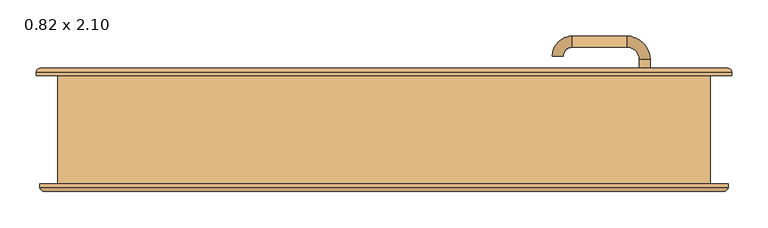
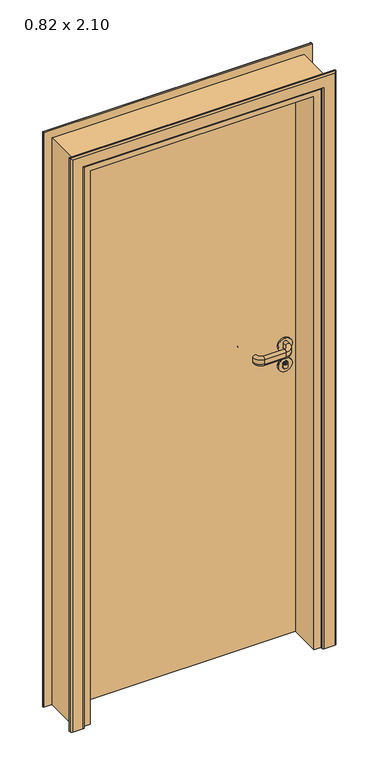
"""IFC4 building model written with IfcOpenShell, lengths in millimetres: door geometry, CC_PORTA ABRIR_1 FOLHA LISA : 0.82 x 2.10."""

import ifcopenshell
import ifcopenshell.guid

model = None  # the IFC model being written
_history = None  # IfcOwnerHistory: only IFC2X3 demands one
_inside = {}  # id of a spatial element -> (the spatial element, [elements in it])
_under = {}  # id of a project, library or spatial element -> (it, [spatial elements below it])
_declared = {}  # id of a project -> (the project, [libraries it declares])
_typed = {}  # id of a type object -> (the type object, [elements of that type])
_made_of = {}  # id of a material, layer set ... -> (it, [elements and type objects made of it])


def new_model(schema):
    """Start an empty IFC model of exactly this schema.

    Asked for "IFC4X3", IfcOpenShell would pick the latest addendum, in which some entities
    have other attributes; the version numbers below select the first issue.
    IFC2X3 requires an IfcOwnerHistory on every rooted entity: one is made here for all.
    """
    global model, _history
    if schema == "IFC4X3":
        model = ifcopenshell.file(schema_version=(4, 3, 0, 0))
    else:
        model = ifcopenshell.file(schema=schema)
    _inside.clear()
    _under.clear()
    _declared.clear()
    _typed.clear()
    _made_of.clear()
    _history = None
    if model.schema == "IFC2X3":
        org = make("IfcOrganization", Name="unknown")
        user = make(
            "IfcPersonAndOrganization",
            ThePerson=make("IfcPerson", FamilyName="unknown"),
            TheOrganization=org,
        )
        app = make(
            "IfcApplication",
            ApplicationDeveloper=org,
            Version="unknown",
            ApplicationFullName="unknown",
            ApplicationIdentifier="unknown",
        )
        _history = make(
            "IfcOwnerHistory",
            OwningUser=user,
            OwningApplication=app,
            ChangeAction="ADDED",
            CreationDate=0,
        )
    return model


def make(cls, **values):
    """One entity of the class cls with the attributes given. An attribute that is None is left unset."""
    return model.create_entity(
        cls, **{name: value for name, value in values.items() if value is not None}
    )


def rooted(cls, **values):
    """An entity with a GlobalId (a new one), such as an element, a storey or a relation."""
    return make(cls, GlobalId=ifcopenshell.guid.new(), OwnerHistory=_history, **values)


def si_unit(unit_type, name, prefix=None):
    """IfcSIUnit, for example si_unit("LENGTHUNIT", "METRE", prefix="MILLI")."""
    return make("IfcSIUnit", UnitType=unit_type, Prefix=prefix, Name=name)


def assignment(units):
    """IfcUnitAssignment: the units of a project."""
    return None if units is None else make("IfcUnitAssignment", Units=units)


def point(xyz):
    """IfcCartesianPoint."""
    return None if xyz is None else make("IfcCartesianPoint", Coordinates=xyz)


def direction(xyz):
    """IfcDirection."""
    return None if xyz is None else make("IfcDirection", DirectionRatios=xyz)


def frame(location, z_axis=None, x_axis=None):
    """IfcAxis2Placement3D, a coordinate frame: its origin and axes. An axis left out is left unset."""
    return make(
        "IfcAxis2Placement3D",
        Location=point(location),
        Axis=direction(z_axis),
        RefDirection=direction(x_axis),
    )


def frame_2d(location, x_axis=None):
    """IfcAxis2Placement2D, a coordinate frame in the plane: its origin and x axis."""
    return make(
        "IfcAxis2Placement2D", Location=point(location), RefDirection=direction(x_axis)
    )


def origin():
    """The frame at (0, 0, 0) with its axes left unset."""
    return frame((0.0, 0.0, 0.0))


def origin_with_axes():
    """The frame at (0, 0, 0) with the z axis (0, 0, 1) and the x axis (1, 0, 0) written out."""
    return frame((0.0, 0.0, 0.0), z_axis=(0.0, 0.0, 1.0), x_axis=(1.0, 0.0, 0.0))


def place(relative_to, where):
    """IfcLocalPlacement: puts the frame where relative to a parent placement (None: the world)."""
    return make(
        "IfcLocalPlacement", PlacementRelTo=relative_to, RelativePlacement=where
    )


def context(
    kind, dimensions, precision=None, world=None, true_north=None, identifier=None
):
    """IfcGeometricRepresentationContext, for example the 3D "Model" context."""
    return make(
        "IfcGeometricRepresentationContext",
        ContextIdentifier=identifier,
        ContextType=kind,
        CoordinateSpaceDimension=dimensions,
        Precision=precision,
        WorldCoordinateSystem=world,
        TrueNorth=true_north,
    )


def project(units=None, contexts=None):
    """IfcProject with its units and contexts."""
    return rooted(
        "IfcProject",
        Name="project",
        RepresentationContexts=contexts,
        UnitsInContext=assignment(units),
    )


def spatial(cls, under=None, at=None, **own):
    """A site, building, storey or space (cls), placed at a placement, below another one or the project."""
    s = rooted(cls, ObjectPlacement=at, **own)
    if under is not None:
        _under.setdefault(under.id(), (under, []))[1].append(s)
    return s


def polyline(points):
    """IfcPolyline through the points."""
    return make("IfcPolyline", Points=[point(p) for p in points])


def circle_curve(where, radius):
    """IfcCircle in the frame where."""
    return make("IfcCircle", Position=where, Radius=radius)


def ellipse_curve(where, semi_axis1, semi_axis2):
    """IfcEllipse in the frame where."""
    return make(
        "IfcEllipse", Position=where, SemiAxis1=semi_axis1, SemiAxis2=semi_axis2
    )


def trimmed(basis, trim1, trim2, sense, master):
    """IfcTrimmedCurve: the piece of a basis curve between two trims."""
    return make(
        "IfcTrimmedCurve",
        BasisCurve=basis,
        Trim1=trim1,
        Trim2=trim2,
        SenseAgreement=sense,
        MasterRepresentation=master,
    )


def segment(curve, same_sense, transition):
    """IfcCompositeCurveSegment."""
    return make(
        "IfcCompositeCurveSegment",
        Transition=transition,
        SameSense=same_sense,
        ParentCurve=curve,
    )


def composite_curve(segments, self_intersect=None):
    """IfcCompositeCurve: segments joined end to end."""
    return make("IfcCompositeCurve", Segments=segments, SelfIntersect=self_intersect)


def outline(outer, holes=None, kind="AREA"):
    """IfcArbitraryClosedProfileDef: a profile drawn as a closed curve; with holes, ...WithVoids."""
    if holes is None:
        return make("IfcArbitraryClosedProfileDef", ProfileType=kind, OuterCurve=outer)
    return make(
        "IfcArbitraryProfileDefWithVoids",
        ProfileType=kind,
        OuterCurve=outer,
        InnerCurves=holes,
    )


def extrude(swept, where, along, depth):
    """IfcExtrudedAreaSolid: the profile swept, set in the frame where, extruded along a direction by depth."""
    return make(
        "IfcExtrudedAreaSolid",
        SweptArea=swept,
        Position=where,
        ExtrudedDirection=direction(along),
        Depth=depth,
    )


def faces_of(points, faces, orient=None, outer=None):
    """IfcFace entities. A face is a list of loops; a loop is a list of indices into points, from 0.

    orient and outer hold one flag for each loop. By default every Orientation is true, the
    first loop of a face is its IfcFaceOuterBound and the others are IfcFaceBound.
    """
    made = []
    for i, loops in enumerate(faces):
        bounds = []
        for j, loop in enumerate(loops):
            is_outer = j == 0 if outer is None else outer[i][j]
            bounds.append(
                make(
                    "IfcFaceOuterBound" if is_outer else "IfcFaceBound",
                    Bound=make("IfcPolyLoop", Polygon=[points[k] for k in loop]),
                    Orientation=True if orient is None else orient[i][j],
                )
            )
        made.append(make("IfcFace", Bounds=bounds))
    return made


def faceted_brep(points, faces, orient=None, outer=None, voids=None):
    """IfcFacetedBrep: a solid bounded by flat faces; with voids (closed shells), ...WithVoids."""
    shared = [point(p) for p in points]
    hull = make("IfcClosedShell", CfsFaces=faces_of(shared, faces, orient, outer))
    if voids is None:
        return make("IfcFacetedBrep", Outer=hull)
    return make(
        "IfcFacetedBrepWithVoids",
        Outer=hull,
        Voids=[
            make(cls, CfsFaces=faces_of(shared, fs, o, b)) for cls, fs, o, b in voids
        ],
    )


def shape(context_of_items, identifier, shape_type, items):
    """IfcShapeRepresentation: the items that make up one representation, for example the "Body"."""
    return make(
        "IfcShapeRepresentation",
        ContextOfItems=context_of_items,
        RepresentationIdentifier=identifier,
        RepresentationType=shape_type,
        Items=items,
    )


def source(mapping_origin, context_of_items, identifier, shape_type, items):
    """IfcRepresentationMap: a shape defined once, which mapped items show again and again."""
    return make(
        "IfcRepresentationMap",
        MappingOrigin=mapping_origin,
        MappedRepresentation=shape(context_of_items, identifier, shape_type, items),
    )


def transform(
    local_origin,
    x_axis=None,
    y_axis=None,
    z_axis=None,
    scale=None,
    scale2=None,
    scale3=None,
    uniform=True,
):
    """IfcCartesianTransformationOperator3D, or its non-uniform kind. x_axis, y_axis, z_axis: its Axis1, 2, 3."""
    if uniform:
        return make(
            "IfcCartesianTransformationOperator3D",
            Axis1=direction(x_axis),
            Axis2=direction(y_axis),
            LocalOrigin=point(local_origin),
            Scale=scale,
            Axis3=direction(z_axis),
        )
    return make(
        "IfcCartesianTransformationOperator3DnonUniform",
        Axis1=direction(x_axis),
        Axis2=direction(y_axis),
        LocalOrigin=point(local_origin),
        Scale=scale,
        Axis3=direction(z_axis),
        Scale2=scale2,
        Scale3=scale3,
    )


def mapped(mapping_source, mapping_target):
    """IfcMappedItem: shows the shape of a source again, moved by a transform."""
    return make(
        "IfcMappedItem", MappingSource=mapping_source, MappingTarget=mapping_target
    )


def made_of(thing, what):
    """Note that an element or type object is made of a material, layer set ...; save() writes the relation."""
    if what is not None:
        _made_of.setdefault(what.id(), (what, []))[1].append(thing)
    return thing


def element(
    cls,
    number,
    at=None,
    inside=None,
    cuts=None,
    type_object=None,
    material=None,
    context=None,
    identifier="Body",
    shape_type=None,
    held_by="IfcProductDefinitionShape",
    body=None,
    shapes=None,
    **own,
):
    """One element of the class cls, such as IfcWall. Its Tag is "e" and its number.

    at: its placement. inside: the storey or other place that contains it. cuts: it is an
    opening in that element (IfcRelVoidsElement). A single representation is given by context,
    identifier, shape_type and body (its items); several are given by shapes. held_by: the class
    of the entity that holds the representations. save() writes the other relations.
    """
    e = rooted(cls, Tag="e%d" % number, ObjectPlacement=at, **own)
    if body is not None:
        shapes = [shape(context, identifier, shape_type, body)]
    if shapes is not None:
        e.Representation = make(held_by, Representations=shapes)
    if inside is not None:
        _inside.setdefault(inside.id(), (inside, []))[1].append(e)
    if cuts is not None:
        rooted(
            "IfcRelVoidsElement", RelatingBuildingElement=cuts, RelatedOpeningElement=e
        )
    if type_object is not None:
        _typed.setdefault(type_object.id(), (type_object, []))[1].append(e)
    return made_of(e, material)


def aggregate(whole, parts):
    """IfcRelAggregates: a whole, such as a stair, and the parts it consists of."""
    return rooted("IfcRelAggregates", RelatingObject=whole, RelatedObjects=parts)


def save(model, path):
    """Write the relations noted so far, then the file.

    IfcRelAggregates (storeys below a building ...), IfcRelContainedInSpatialStructure (elements
    in a storey), IfcRelDefinesByType, IfcRelAssociatesMaterial and IfcRelDeclares: one each for
    every whole, place, type object, material and project.
    """
    for whole, parts in _under.values():
        aggregate(whole, parts)
    for where, things in _inside.values():
        rooted(
            "IfcRelContainedInSpatialStructure",
            RelatedElements=things,
            RelatingStructure=where,
        )
    for kind, things in _typed.values():
        rooted("IfcRelDefinesByType", RelatedObjects=things, RelatingType=kind)
    for what, things in _made_of.values():
        rooted("IfcRelAssociatesMaterial", RelatedObjects=things, RelatingMaterial=what)
    for by, libraries in _declared.values():
        rooted("IfcRelDeclares", RelatingContext=by, RelatedDefinitions=libraries)
    model.write(path)


def plane_surface(at):
    """IfcPlane: the flat surface through the origin of the frame at, square to its z axis."""
    return make("IfcPlane", Position=at)


def cylinder_surface(at, radius):
    """IfcCylindricalSurface: all points at the distance radius from the z axis of the frame at."""
    return make("IfcCylindricalSurface", Position=at, Radius=radius)


def revolved_surface(curve, axis_point, axis_direction):
    """IfcSurfaceOfRevolution: the curve turned about the line through axis_point along axis_direction."""
    return make(
        "IfcSurfaceOfRevolution",
        SweptCurve=make("IfcArbitraryOpenProfileDef", ProfileType="CURVE", Curve=curve),
        AxisPosition=make("IfcAxis1Placement", Location=point(axis_point), Axis=direction(axis_direction)),
    )


def advanced_brep(points, edges, surfaces, faces):
    """IfcAdvancedBrep: a solid bounded by faces that lie on surfaces and meet in shared edges.

    An edge is (start, end): straight between two places in points (the first is 0);
    or (start, end, curve); or (start, end, curve, False) where it runs against its curve.
    A face is (place in surfaces, loops), or (place, loops, False) where it looks against
    its surface's normal. A loop lists edges by number (the first is 1), with a minus sign
    where the edge is run from its end to its start. The first loop is the outer one.
    """
    corners = [point(p) for p in points]
    vertices = [make("IfcVertexPoint", VertexGeometry=c) for c in corners]
    made = []
    for start, end, *more in edges:
        made.append(
            make(
                "IfcEdgeCurve",
                EdgeStart=vertices[start],
                EdgeEnd=vertices[end],
                EdgeGeometry=more[0] if more else make("IfcPolyline", Points=[corners[start], corners[end]]),
                SameSense=more[1] if len(more) > 1 else True,
            )
        )
    hull = []
    for where, loops, *sense in faces:
        bounds = []
        for j, loop in enumerate(loops):
            ring = [make("IfcOrientedEdge", EdgeElement=made[abs(k) - 1], Orientation=k > 0) for k in loop]
            bounds.append(
                make(
                    "IfcFaceOuterBound" if j == 0 else "IfcFaceBound",
                    Bound=make("IfcEdgeLoop", EdgeList=ring),
                    Orientation=True,
                )
            )
        hull.append(make("IfcAdvancedFace", Bounds=bounds, FaceSurface=surfaces[where], SameSense=sense[0] if sense else True))
    return make("IfcAdvancedBrep", Outer=make("IfcClosedShell", CfsFaces=hull))


def door_0_82_x_2_10_9ce577dd(model_context):
    return source(origin(), model_context, "Body", "SolidModel", [
        advanced_brep(
        [(352.5, 40.0, 1091.5062746), (352.5, 40.0, 1108.3826844), (367.5, 40.0, 1108.3826844), (367.5, 40.0, 1091.5062746), (367.5, 18.0, 1108.3826844), (367.5, 18.0, 1091.5062746), (352.5, 18.0, 1091.5062746), (352.5, 18.0, 1108.3826844), (335.0, -14.5, 1108.3826844), (260.0, -14.5, 1108.3826844), (260.0, -14.5, 1091.5062746), (335.0, -14.5, 1091.5062746), (335.0, 0.5, 1091.5062746), (260.0, 0.5, 1091.5062746), (260.0, 0.5, 1108.3826844), (335.0, 0.5, 1108.3826844), (247.5, 13.0, 1091.5062746), (232.5, 13.0, 1091.5062746), (232.5, 13.0, 1108.3826844), (247.5, 13.0, 1108.3826844)],
        [
            (0, 1),
            (1, 2, circle_curve(frame((360.0, 40.0, 1108.3826844), z_axis=(0.0, 1.0, 0.0), x_axis=(0.0, 0.0, 1.0)), 7.5)),
            (2, 3),
            (3, 0, circle_curve(frame((360.0, 40.0, 1091.5062746), z_axis=(0.0, 1.0, 0.0), x_axis=(0.0, 0.0, 1.0)), 7.5)),
            (2, 4),
            (4, 5),
            (5, 3),
            (0, 6),
            (6, 7),
            (7, 1),
            (8, 9),
            (9, 10),
            (10, 11),
            (11, 8),
            (12, 13),
            (13, 14),
            (14, 15),
            (15, 12),
            (5, 6, circle_curve(frame((360.0, 18.0, 1091.5062746), z_axis=(0.0, 1.0, 0.0), x_axis=(0.0, 0.0, 1.0)), 7.5)),
            (7, 4, circle_curve(frame((360.0, 18.0, 1108.3826844), z_axis=(0.0, 1.0, 0.0), x_axis=(0.0, 0.0, 1.0)), 7.5)),
            (10, 13, circle_curve(frame((260.0, -7.0, 1091.5062746), z_axis=(1.0, 0.0, 0.0), x_axis=(0.0, 0.0, 1.0)), 7.5)),
            (12, 11, circle_curve(frame((335.0, -7.0, 1091.5062746), z_axis=(-1.0, 0.0, 0.0), x_axis=(0.0, 0.0, 1.0)), 7.5)),
            (14, 9, circle_curve(frame((260.0, -7.0, 1108.3826844), z_axis=(1.0, 0.0, 0.0), x_axis=(0.0, 0.0, 1.0)), 7.5)),
            (8, 15, circle_curve(frame((335.0, -7.0, 1108.3826844), z_axis=(-1.0, 0.0, 0.0), x_axis=(0.0, 0.0, 1.0)), 7.5)),
            (12, 6, circle_curve(frame((335.0, 18.0, 1091.5062746), z_axis=(0.0, 0.0, 1.0), x_axis=(1.0, 0.0, 0.0)), 17.5)),
            (5, 11, circle_curve(frame((335.0, 18.0, 1091.5062746), z_axis=(0.0, 0.0, -1.0), x_axis=(1.0, 0.0, 0.0)), 32.5)),
            (4, 8, circle_curve(frame((335.0, 18.0, 1108.3826844), z_axis=(0.0, 0.0, -1.0), x_axis=(1.0, 0.0, 0.0)), 32.5)),
            (7, 15, circle_curve(frame((335.0, 18.0, 1108.3826844), z_axis=(0.0, 0.0, -1.0), x_axis=(1.0, 0.0, 0.0)), 17.5)),
            (16, 17, circle_curve(frame((240.0, 13.0, 1091.5062746), z_axis=(0.0, 1.0, 0.0), x_axis=(0.0, 0.0, 1.0)), 7.5)),
            (17, 18),
            (18, 19, circle_curve(frame((240.0, 13.0, 1108.3826844), z_axis=(0.0, 1.0, 0.0), x_axis=(0.0, 0.0, 1.0)), 7.5)),
            (19, 16),
            (16, 13, circle_curve(frame((260.0, 13.0, 1091.5062746), z_axis=(0.0, 0.0, 1.0), x_axis=(0.0, -1.0, 0.0)), 12.5)),
            (10, 17, circle_curve(frame((260.0, 13.0, 1091.5062746), z_axis=(0.0, 0.0, -1.0), x_axis=(0.0, -1.0, 0.0)), 27.5)),
            (9, 18, circle_curve(frame((260.0, 13.0, 1108.3826844), z_axis=(0.0, 0.0, -1.0), x_axis=(0.0, -1.0, 0.0)), 27.5)),
            (14, 19, circle_curve(frame((260.0, 13.0, 1108.3826844), z_axis=(0.0, 0.0, -1.0), x_axis=(0.0, -1.0, 0.0)), 12.5)),
        ],
        [
            plane_surface(frame((360.0, 40.0, 1099.9444795), z_axis=(0.0, 1.0, 0.0), x_axis=(0.0, 0.0, 1.0))),
            plane_surface(frame((367.5, 40.0, 1091.5062746), z_axis=(1.0, 0.0, 0.0), x_axis=(0.0, -1.0, 0.0))),
            plane_surface(frame((352.5, 40.0, 1108.3826844), z_axis=(-1.0, 0.0, 0.0), x_axis=(0.0, -1.0, 0.0))),
            plane_surface(frame((335.0, -14.5, 1091.5062746), z_axis=(0.0, -1.0, 0.0), x_axis=(-1.0, 0.0, 0.0))),
            plane_surface(frame((335.0, 0.5, 1108.3826844), z_axis=(0.0, 1.0, 0.0), x_axis=(-1.0, 0.0, 0.0))),
            cylinder_surface(frame((360.0, 40.0, 1091.5062746), z_axis=(0.0, 1.0, 0.0), x_axis=(0.0, 0.0, 1.0)), 7.5),
            cylinder_surface(frame((360.0, 40.0, 1108.3826844), z_axis=(0.0, 1.0, 0.0), x_axis=(0.0, 0.0, 1.0)), 7.5),
            cylinder_surface(frame((335.0, -7.0, 1091.5062746), z_axis=(1.0, 0.0, 0.0), x_axis=(0.0, 0.0, 1.0)), 7.5),
            cylinder_surface(frame((335.0, -7.0, 1108.3826844), z_axis=(1.0, 0.0, 0.0), x_axis=(0.0, 0.0, 1.0)), 7.5),
            revolved_surface(trimmed(ellipse_curve(frame((360.0, 18.0, 1091.5062746), z_axis=(0.0, -1.0, 0.0), x_axis=(0.0, 0.0, 1.0)), 7.5, 7.5), [point((352.5, 18.0, 1091.5062746))], [point((367.5, 18.0, 1091.5062746))], True, "CARTESIAN"), (335.0, 18.0, 1099.9444795), (0.0, 0.0, 1.0)),
            cylinder_surface(frame((335.0, 18.0, 1099.9444795), z_axis=(0.0, 0.0, 1.0), x_axis=(1.0, 0.0, 0.0)), 32.5),
            revolved_surface(trimmed(ellipse_curve(frame((360.0, 18.0, 1108.3826844), z_axis=(0.0, -1.0, 0.0), x_axis=(0.0, 0.0, 1.0)), 7.5, 7.5), [point((367.5, 18.0, 1108.3826844))], [point((352.5, 18.0, 1108.3826844))], True, "CARTESIAN"), (335.0, 18.0, 1099.9444795), (0.0, 0.0, 1.0)),
            revolved_surface(polyline([(352.5, 18.0, 1108.3826844), (352.5, 18.0, 1091.5062746)]), (335.0, 18.0, 1099.9444795), (0.0, 0.0, 1.0)),
            plane_surface(frame((240.0, 13.0, 1099.9444795), z_axis=(0.0, 1.0, 0.0), x_axis=(0.0, 0.0, 1.0))),
            revolved_surface(trimmed(ellipse_curve(frame((260.0, -7.0, 1091.5062746), z_axis=(-1.0, 0.0, 0.0), x_axis=(0.0, 0.0, 1.0)), 7.5, 7.5), [point((260.0, 0.5, 1091.5062746))], [point((260.0, -14.5, 1091.5062746))], True, "CARTESIAN"), (260.0, 13.0, 1099.9444795), (0.0, 0.0, 1.0)),
            cylinder_surface(frame((260.0, 13.0, 1099.9444795), z_axis=(0.0, 0.0, 1.0), x_axis=(0.0, -1.0, 0.0)), 27.5),
            revolved_surface(trimmed(ellipse_curve(frame((260.0, -7.0, 1108.3826844), z_axis=(-1.0, 0.0, 0.0), x_axis=(0.0, 0.0, 1.0)), 7.5, 7.5), [point((260.0, -14.5, 1108.3826844))], [point((260.0, 0.5, 1108.3826844))], True, "CARTESIAN"), (260.0, 13.0, 1099.9444795), (0.0, 0.0, 1.0)),
            revolved_surface(polyline([(260.0, 0.5, 1108.3826844), (260.0, 0.5, 1091.5062746)]), (260.0, 13.0, 1099.9444795), (0.0, 0.0, 1.0)),
        ],
        [
            (0, [[1, 2, 3, 4]]),
            (1, [[5, 6, 7, -3]]),
            (2, [[8, 9, 10, -1]]),
            (3, [[11, 12, 13, 14]]),
            (4, [[15, 16, 17, 18]]),
            (5, [[-7, 19, -8, -4]]),
            (6, [[-10, 20, -5, -2]]),
            (7, [[-13, 21, -15, 22]]),
            (8, [[-17, 23, -11, 24]]),
            (9, [[-22, 25, -19, 26]]),
            (10, [[-14, -26, -6, 27]]),
            (11, [[-24, -27, -20, 28]]),
            (12, [[-18, -28, -9, -25]]),
            (13, [[29, 30, 31, 32]]),
            (14, [[-29, 33, -21, 34]]),
            (15, [[-30, -34, -12, 35]]),
            (16, [[-31, -35, -23, 36]]),
            (17, [[-32, -36, -16, -33]]),
        ],
    ),
        extrude(outline(polyline([(361.0, 40.0), (361.0, 30.9), (359.0, 30.9), (359.0, 40.0), (361.0, 40.0)])), frame((0.0, 0.0, 1027.9555433), z_axis=(0.0, 0.0, 1.0), x_axis=(1.0, 0.0, 0.0)), (0.0, 0.0, 1.0), 7.8071257),
        extrude(outline(composite_curve([segment(trimmed(circle_curve(frame_2d((1031.5611613, 360.0)), 5.0), [point((1036.5611613, 360.0))], [point((1026.5611613, 360.0))], False, "CARTESIAN"), True, "CONTINUOUS"), segment(trimmed(circle_curve(frame_2d((1031.5611613, 360.0)), 5.0), [point((1026.5611613, 360.0))], [point((1036.5611613, 360.0))], False, "CARTESIAN"), True, "CONTINUOUS")], self_intersect=False), holes=[polyline([(1035.7626689, 361.0), (1027.9555433, 361.0), (1027.9555433, 359.0), (1035.7626689, 359.0), (1035.7626689, 361.0)])]), frame((0.0, 30.0, 0.0), z_axis=(0.0, 1.0, 0.0), x_axis=(0.0, 0.0, 1.0)), (0.0, 0.0, 1.0), 10.0),
        extrude(outline(composite_curve([segment(polyline([(1033.4817325, 352.5), (1016.4817325, 352.5)]), True, "CONTINUOUS"), segment(trimmed(circle_curve(frame_2d((1016.4817325, 356.5)), 4.0), [point((1016.4817325, 352.5))], [point((1012.4817325, 356.5))], False, "CARTESIAN"), True, "CONTINUOUS"), segment(polyline([(1012.4817325, 356.5), (1012.4817325, 363.5)]), True, "CONTINUOUS"), segment(trimmed(circle_curve(frame_2d((1016.4817325, 363.5)), 4.0), [point((1012.4817325, 363.5))], [point((1016.4817325, 367.5))], False, "CARTESIAN"), True, "CONTINUOUS"), segment(polyline([(1016.4817325, 367.5), (1033.4817325, 367.5)]), True, "CONTINUOUS"), segment(trimmed(circle_curve(frame_2d((1033.4817325, 363.5)), 4.0), [point((1033.4817325, 367.5))], [point((1037.4817325, 363.5))], False, "CARTESIAN"), True, "CONTINUOUS"), segment(polyline([(1037.4817325, 363.5), (1037.4817325, 356.5)]), True, "CONTINUOUS"), segment(trimmed(circle_curve(frame_2d((1033.4817325, 356.5)), 4.0), [point((1037.4817325, 356.5))], [point((1033.4817325, 352.5))], False, "CARTESIAN"), True, "CONTINUOUS")], self_intersect=False)), frame((0.0, 31.0, 0.0), z_axis=(0.0, 1.0, 0.0), x_axis=(0.0, 0.0, 1.0)), (0.0, 0.0, 1.0), 9.0),
        extrude(outline(composite_curve([segment(trimmed(circle_curve(frame_2d((1099.9444795, 360.0)), 25.0), [point((1124.9444795, 360.0))], [point((1074.9444795, 360.0))], False, "CARTESIAN"), True, "CONTINUOUS"), segment(trimmed(circle_curve(frame_2d((1099.9444795, 360.0)), 25.0), [point((1074.9444795, 360.0))], [point((1124.9444795, 360.0))], False, "CARTESIAN"), True, "CONTINUOUS")], self_intersect=False)), frame((0.0, 34.0, 0.0), z_axis=(0.0, 1.0, 0.0), x_axis=(0.0, 0.0, 1.0)), (0.0, 0.0, 1.0), 6.0),
        extrude(outline(composite_curve([segment(trimmed(circle_curve(frame_2d((1024.9444795, 360.0)), 25.0), [point((1049.9444795, 360.0))], [point((999.9444795, 360.0))], False, "CARTESIAN"), True, "CONTINUOUS"), segment(trimmed(circle_curve(frame_2d((1024.9444795, 360.0)), 25.0), [point((999.9444795, 360.0))], [point((1049.9444795, 360.0))], False, "CARTESIAN"), True, "CONTINUOUS")], self_intersect=False), holes=[composite_curve([segment(trimmed(circle_curve(frame_2d((1033.4817325, 363.5)), 4.0), [point((1037.4817325, 363.5))], [point((1033.4817325, 367.5))], True, "CARTESIAN"), True, "CONTINUOUS"), segment(polyline([(1033.4817325, 367.5), (1016.4817325, 367.5)]), True, "CONTINUOUS"), segment(trimmed(circle_curve(frame_2d((1016.4817325, 363.5)), 4.0), [point((1016.4817325, 367.5))], [point((1012.4817325, 363.5))], True, "CARTESIAN"), True, "CONTINUOUS"), segment(polyline([(1012.4817325, 363.5), (1012.4817325, 356.5)]), True, "CONTINUOUS"), segment(trimmed(circle_curve(frame_2d((1016.4817325, 356.5)), 4.0), [point((1012.4817325, 356.5))], [point((1016.4817325, 352.5))], True, "CARTESIAN"), True, "CONTINUOUS"), segment(polyline([(1016.4817325, 352.5), (1033.4817325, 352.5)]), True, "CONTINUOUS"), segment(trimmed(circle_curve(frame_2d((1033.4817325, 356.5)), 4.0), [point((1033.4817325, 352.5))], [point((1037.4817325, 356.5))], True, "CARTESIAN"), True, "CONTINUOUS"), segment(polyline([(1037.4817325, 356.5), (1037.4817325, 363.5)]), True, "CONTINUOUS")], self_intersect=False)]), frame((0.0, 34.0, 0.0), z_axis=(0.0, 1.0, 0.0), x_axis=(0.0, 0.0, 1.0)), (0.0, 0.0, 1.0), 6.0),
        extrude(outline(polyline([(361.0, 84.1), (361.0, 75.0), (359.0, 75.0), (359.0, 84.1), (361.0, 84.1)])), frame((0.0, 0.0, 1027.9555433), z_axis=(0.0, 0.0, 1.0), x_axis=(1.0, 0.0, 0.0)), (0.0, 0.0, 1.0), 7.8071257),
        advanced_brep(
        [(360.0, 85.0, 1036.5611613), (360.0, 85.0, 1026.5611613), (361.0, 85.0, 1035.7626689), (359.0, 85.0, 1035.7626689), (359.0, 85.0, 1027.9555433), (361.0, 85.0, 1027.9555433), (360.0, 75.0, 1049.9444795), (360.0, 75.0, 999.9444795), (360.0, 84.0, 1026.5611613), (360.0, 84.0, 1036.5611613), (361.0, 84.0, 1027.9555433), (361.0, 84.0, 1035.7626689), (359.0, 84.0, 1027.9555433), (359.0, 84.0, 1035.7626689), (352.5, 84.0, 1033.4817325), (356.5, 84.0, 1037.4817325), (363.5, 84.0, 1037.4817325), (367.5, 84.0, 1033.4817325), (367.5, 84.0, 1016.4817325), (363.5, 84.0, 1012.4817325), (356.5, 84.0, 1012.4817325), (352.5, 84.0, 1016.4817325), (352.5, 81.0, 1016.4817325), (352.5, 81.0, 1033.4817325), (356.5, 81.0, 1012.4817325), (363.5, 81.0, 1012.4817325), (367.5, 81.0, 1016.4817325), (367.5, 81.0, 1033.4817325), (363.5, 81.0, 1037.4817325), (356.5, 81.0, 1037.4817325), (360.0, 81.0, 1049.9444795), (360.0, 81.0, 999.9444795)],
        [
            (0, 1, circle_curve(frame((360.0, 85.0, 1031.5611613), z_axis=(0.0, 1.0, 0.0), x_axis=(0.0, 0.0, -1.0)), 5.0)),
            (1, 0, circle_curve(frame((360.0, 85.0, 1031.5611613), z_axis=(0.0, 1.0, 0.0), x_axis=(0.0, 0.0, -1.0)), 5.0)),
            (2, 3),
            (3, 4),
            (4, 5),
            (5, 2),
            (6, 7, circle_curve(frame((360.0, 75.0, 1024.9444795), z_axis=(0.0, -1.0, 0.0), x_axis=(0.0, 0.0, -1.0)), 25.0)),
            (7, 6, circle_curve(frame((360.0, 75.0, 1024.9444795), z_axis=(0.0, -1.0, 0.0), x_axis=(0.0, 0.0, -1.0)), 25.0)),
            (1, 8),
            (8, 9, circle_curve(frame((360.0, 84.0, 1031.5611613), z_axis=(0.0, 1.0, 0.0), x_axis=(0.0, 0.0, -1.0)), 5.0)),
            (9, 0),
            (9, 8, circle_curve(frame((360.0, 84.0, 1031.5611613), z_axis=(0.0, 1.0, 0.0), x_axis=(0.0, 0.0, -1.0)), 5.0)),
            (5, 10),
            (10, 11),
            (11, 2),
            (4, 12),
            (12, 10),
            (3, 13),
            (13, 12),
            (11, 13),
            (14, 15, circle_curve(frame((356.5, 84.0, 1033.4817325), z_axis=(0.0, 1.0, 0.0), x_axis=(0.0, 0.0, -1.0)), 4.0)),
            (15, 16),
            (16, 17, circle_curve(frame((363.5, 84.0, 1033.4817325), z_axis=(0.0, 1.0, 0.0), x_axis=(0.0, 0.0, -1.0)), 4.0)),
            (17, 18),
            (18, 19, circle_curve(frame((363.5, 84.0, 1016.4817325), z_axis=(0.0, 1.0, 0.0), x_axis=(0.0, 0.0, -1.0)), 4.0)),
            (19, 20),
            (20, 21, circle_curve(frame((356.5, 84.0, 1016.4817325), z_axis=(0.0, 1.0, 0.0), x_axis=(0.0, 0.0, -1.0)), 4.0)),
            (21, 14),
            (21, 22),
            (22, 23),
            (23, 14),
            (20, 24),
            (24, 22, circle_curve(frame((356.5, 81.0, 1016.4817325), z_axis=(0.0, 1.0, 0.0), x_axis=(0.0, 0.0, -1.0)), 4.0)),
            (19, 25),
            (25, 24),
            (18, 26),
            (26, 25, circle_curve(frame((363.5, 81.0, 1016.4817325), z_axis=(0.0, 1.0, 0.0), x_axis=(0.0, 0.0, -1.0)), 4.0)),
            (17, 27),
            (27, 26),
            (16, 28),
            (28, 27, circle_curve(frame((363.5, 81.0, 1033.4817325), z_axis=(0.0, 1.0, 0.0), x_axis=(0.0, 0.0, -1.0)), 4.0)),
            (15, 29),
            (29, 28),
            (23, 29, circle_curve(frame((356.5, 81.0, 1033.4817325), z_axis=(0.0, 1.0, 0.0), x_axis=(0.0, 0.0, -1.0)), 4.0)),
            (30, 31, circle_curve(frame((360.0, 81.0, 1024.9444795), z_axis=(0.0, 1.0, 0.0), x_axis=(0.0, 0.0, -1.0)), 25.0)),
            (31, 30, circle_curve(frame((360.0, 81.0, 1024.9444795), z_axis=(0.0, 1.0, 0.0), x_axis=(0.0, 0.0, -1.0)), 25.0)),
            (31, 7),
            (6, 30),
        ],
        [
            plane_surface(frame((360.0, 85.0, 1026.5611613), z_axis=(0.0, 1.0, 0.0), x_axis=(1.0, 0.0, 0.0))),
            plane_surface(frame((360.0, 75.0, 1026.5611613), z_axis=(0.0, -1.0, 0.0), x_axis=(-1.0, 0.0, 0.0))),
            cylinder_surface(frame((360.0, 75.0, 1031.5611613), z_axis=(0.0, 1.0, 0.0), x_axis=(0.0, 0.0, -1.0)), 5.0),
            plane_surface(frame((361.0, 85.0, 1035.7626689), z_axis=(-1.0, 0.0, 0.0), x_axis=(0.0, -1.0, 0.0))),
            plane_surface(frame((361.0, 85.0, 1027.9555433), z_axis=(0.0, 0.0, 1.0), x_axis=(0.0, -1.0, 0.0))),
            plane_surface(frame((359.0, 85.0, 1027.9555433), z_axis=(1.0, 0.0, 0.0), x_axis=(0.0, -1.0, 0.0))),
            plane_surface(frame((359.0, 85.0, 1035.7626689), z_axis=(0.0, 0.0, -1.0), x_axis=(0.0, -1.0, 0.0))),
            plane_surface(frame((352.5, 84.0, 1016.4817325), z_axis=(0.0, 1.0, 0.0), x_axis=(0.0, 0.0, -1.0))),
            plane_surface(frame((352.5, 84.0, 1033.4817325), z_axis=(-1.0, 0.0, 0.0), x_axis=(0.0, -1.0, 0.0))),
            cylinder_surface(frame((356.5, 75.0, 1016.4817325), z_axis=(0.0, 1.0, 0.0), x_axis=(0.0, 0.0, -1.0)), 4.0),
            plane_surface(frame((356.5, 84.0, 1012.4817325), z_axis=(0.0, 0.0, -1.0), x_axis=(0.0, -1.0, 0.0))),
            cylinder_surface(frame((363.5, 75.0, 1016.4817325), z_axis=(0.0, 1.0, 0.0), x_axis=(0.0, 0.0, -1.0)), 4.0),
            plane_surface(frame((367.5, 84.0, 1016.4817325), z_axis=(1.0, 0.0, 0.0), x_axis=(0.0, -1.0, 0.0))),
            cylinder_surface(frame((363.5, 75.0, 1033.4817325), z_axis=(0.0, 1.0, 0.0), x_axis=(0.0, 0.0, -1.0)), 4.0),
            plane_surface(frame((363.5, 84.0, 1037.4817325), z_axis=(0.0, 0.0, 1.0), x_axis=(0.0, -1.0, 0.0))),
            cylinder_surface(frame((356.5, 75.0, 1033.4817325), z_axis=(0.0, 1.0, 0.0), x_axis=(0.0, 0.0, -1.0)), 4.0),
            plane_surface(frame((360.0, 81.0, 1074.9444795), z_axis=(0.0, 1.0, 0.0), x_axis=(1.0, 0.0, 0.0))),
            cylinder_surface(frame((360.0, 75.0, 1024.9444795), z_axis=(0.0, 1.0, 0.0), x_axis=(0.0, 0.0, -1.0)), 25.0),
        ],
        [
            (0, [[1, 2], [3, 4, 5, 6]]),
            (1, [[7, 8]]),
            (2, [[9, 10, 11, -2]]),
            (2, [[-11, 12, -9, -1]]),
            (3, [[13, 14, 15, -6]]),
            (4, [[16, 17, -13, -5]]),
            (5, [[18, 19, -16, -4]]),
            (6, [[-15, 20, -18, -3]]),
            (7, [[-17, -19, -20, -14]]),
            (7, [[21, 22, 23, 24, 25, 26, 27, 28], [-12, -10]]),
            (8, [[29, 30, 31, -28]]),
            (9, [[32, 33, -29, -27]]),
            (10, [[34, 35, -32, -26]]),
            (11, [[36, 37, -34, -25]]),
            (12, [[38, 39, -36, -24]]),
            (13, [[40, 41, -38, -23]]),
            (14, [[42, 43, -40, -22]]),
            (15, [[-31, 44, -42, -21]]),
            (16, [[45, 46], [-33, -35, -37, -39, -41, -43, -44, -30]]),
            (17, [[47, -7, 48, -46]]),
            (17, [[-48, -8, -47, -45]]),
        ],
    ),
        advanced_brep(
        [(360.0, 75.0, 1124.9444795), (360.0, 75.0, 1074.9444795), (360.0, 81.0, 1124.9444795), (360.0, 81.0, 1074.9444795)],
        [
            (0, 1, circle_curve(frame((360.0, 75.0, 1099.9444795), z_axis=(0.0, -1.0, 0.0), x_axis=(0.0, 0.0, -1.0)), 25.0)),
            (1, 0, circle_curve(frame((360.0, 75.0, 1099.9444795), z_axis=(0.0, -1.0, 0.0), x_axis=(0.0, 0.0, -1.0)), 25.0)),
            (2, 3, circle_curve(frame((360.0, 81.0, 1099.9444795), z_axis=(0.0, 1.0, 0.0), x_axis=(0.0, 0.0, -1.0)), 25.0)),
            (3, 2, circle_curve(frame((360.0, 81.0, 1099.9444795), z_axis=(0.0, 1.0, 0.0), x_axis=(0.0, 0.0, -1.0)), 25.0)),
            (3, 1),
            (0, 2),
        ],
        [
            plane_surface(frame((360.0, 75.0, 1026.5611613), z_axis=(0.0, -1.0, 0.0), x_axis=(-1.0, 0.0, 0.0))),
            plane_surface(frame((360.0, 81.0, 1074.9444795), z_axis=(0.0, 1.0, 0.0), x_axis=(1.0, 0.0, 0.0))),
            cylinder_surface(frame((360.0, 75.0, 1099.9444795), z_axis=(0.0, 1.0, 0.0), x_axis=(0.0, 0.0, -1.0)), 25.0),
        ],
        [
            (0, [[1, 2]]),
            (1, [[3, 4]]),
            (2, [[5, -1, 6, -4]]),
            (2, [[-6, -2, -5, -3]]),
        ],
    ),
        advanced_brep(
        [(352.5, 75.0, 1108.4382049), (352.5, 75.0, 1091.5617951), (367.5, 75.0, 1091.5617951), (367.5, 75.0, 1108.4382049), (367.5, 97.0, 1091.5617951), (367.5, 97.0, 1108.4382049), (352.5, 97.0, 1108.4382049), (352.5, 97.0, 1091.5617951), (335.0, 129.5, 1091.5617951), (260.0, 129.5, 1091.5617951), (260.0, 129.5, 1108.4382049), (335.0, 129.5, 1108.4382049), (335.0, 114.5, 1108.4382049), (260.0, 114.5, 1108.4382049), (260.0, 114.5, 1091.5617951), (335.0, 114.5, 1091.5617951), (247.5, 102.0, 1108.4382049), (232.5, 102.0, 1108.4382049), (232.5, 102.0, 1091.5617951), (247.5, 102.0, 1091.5617951)],
        [
            (0, 1),
            (1, 2, circle_curve(frame((360.0, 75.0, 1091.5617951), z_axis=(0.0, -1.0, 0.0), x_axis=(-1.0, 0.0, 0.0)), 7.5)),
            (2, 3),
            (3, 0, circle_curve(frame((360.0, 75.0, 1108.4382049), z_axis=(0.0, -1.0, 0.0), x_axis=(-1.0, 0.0, 0.0)), 7.5)),
            (2, 4),
            (4, 5),
            (5, 3),
            (0, 6),
            (6, 7),
            (7, 1),
            (8, 9),
            (9, 10),
            (10, 11),
            (11, 8),
            (12, 13),
            (13, 14),
            (14, 15),
            (15, 12),
            (5, 6, circle_curve(frame((360.0, 97.0, 1108.4382049), z_axis=(0.0, -1.0, 0.0), x_axis=(-1.0, 0.0, 0.0)), 7.5)),
            (7, 4, circle_curve(frame((360.0, 97.0, 1091.5617951), z_axis=(0.0, -1.0, 0.0), x_axis=(-1.0, 0.0, 0.0)), 7.5)),
            (10, 13, circle_curve(frame((260.0, 122.0, 1108.4382049), z_axis=(1.0, 0.0, 0.0), x_axis=(0.0, -1.0, 0.0)), 7.5)),
            (12, 11, circle_curve(frame((335.0, 122.0, 1108.4382049), z_axis=(-1.0, 0.0, 0.0), x_axis=(0.0, -1.0, 0.0)), 7.5)),
            (14, 9, circle_curve(frame((260.0, 122.0, 1091.5617951), z_axis=(1.0, 0.0, 0.0), x_axis=(0.0, -1.0, 0.0)), 7.5)),
            (8, 15, circle_curve(frame((335.0, 122.0, 1091.5617951), z_axis=(-1.0, 0.0, 0.0), x_axis=(0.0, -1.0, 0.0)), 7.5)),
            (12, 6, circle_curve(frame((335.0, 97.0, 1108.4382049), z_axis=(0.0, 0.0, -1.0), x_axis=(1.0, 0.0, 0.0)), 17.5)),
            (5, 11, circle_curve(frame((335.0, 97.0, 1108.4382049), z_axis=(0.0, 0.0, 1.0), x_axis=(1.0, 0.0, 0.0)), 32.5)),
            (4, 8, circle_curve(frame((335.0, 97.0, 1091.5617951), z_axis=(0.0, 0.0, 1.0), x_axis=(1.0, 0.0, 0.0)), 32.5)),
            (7, 15, circle_curve(frame((335.0, 97.0, 1091.5617951), z_axis=(0.0, 0.0, 1.0), x_axis=(1.0, 0.0, 0.0)), 17.5)),
            (16, 17, circle_curve(frame((240.0, 102.0, 1108.4382049), z_axis=(0.0, -1.0, 0.0), x_axis=(1.0, 0.0, 0.0)), 7.5)),
            (17, 18),
            (18, 19, circle_curve(frame((240.0, 102.0, 1091.5617951), z_axis=(0.0, -1.0, 0.0), x_axis=(1.0, 0.0, 0.0)), 7.5)),
            (19, 16),
            (16, 13, circle_curve(frame((260.0, 102.0, 1108.4382049), z_axis=(0.0, 0.0, -1.0), x_axis=(0.0, 1.0, 0.0)), 12.5)),
            (10, 17, circle_curve(frame((260.0, 102.0, 1108.4382049), z_axis=(0.0, 0.0, 1.0), x_axis=(0.0, 1.0, 0.0)), 27.5)),
            (9, 18, circle_curve(frame((260.0, 102.0, 1091.5617951), z_axis=(0.0, 0.0, 1.0), x_axis=(0.0, 1.0, 0.0)), 27.5)),
            (14, 19, circle_curve(frame((260.0, 102.0, 1091.5617951), z_axis=(0.0, 0.0, 1.0), x_axis=(0.0, 1.0, 0.0)), 12.5)),
        ],
        [
            plane_surface(frame((360.0, 75.0, 1100.0), z_axis=(0.0, -1.0, 0.0), x_axis=(0.0, 0.0, -1.0))),
            plane_surface(frame((367.5, 75.0, 1108.4382049), z_axis=(1.0, 0.0, 0.0), x_axis=(0.0, 1.0, 0.0))),
            plane_surface(frame((352.5, 75.0, 1091.5617951), z_axis=(-1.0, 0.0, 0.0), x_axis=(0.0, 1.0, 0.0))),
            plane_surface(frame((335.0, 129.5, 1108.4382049), z_axis=(0.0, 1.0, 0.0), x_axis=(-1.0, 0.0, 0.0))),
            plane_surface(frame((335.0, 114.5, 1091.5617951), z_axis=(0.0, -1.0, 0.0), x_axis=(-1.0, 0.0, 0.0))),
            cylinder_surface(frame((360.0, 75.0, 1108.4382049), z_axis=(0.0, -1.0, 0.0), x_axis=(-1.0, 0.0, 0.0)), 7.5),
            cylinder_surface(frame((360.0, 75.0, 1091.5617951), z_axis=(0.0, -1.0, 0.0), x_axis=(-1.0, 0.0, 0.0)), 7.5),
            cylinder_surface(frame((335.0, 122.0, 1108.4382049), z_axis=(1.0, 0.0, 0.0), x_axis=(0.0, -1.0, 0.0)), 7.5),
            cylinder_surface(frame((335.0, 122.0, 1091.5617951), z_axis=(1.0, 0.0, 0.0), x_axis=(0.0, -1.0, 0.0)), 7.5),
            revolved_surface(trimmed(ellipse_curve(frame((360.0, 97.0, 1108.4382049), z_axis=(0.0, 1.0, 0.0), x_axis=(-1.0, 0.0, 0.0)), 7.5, 7.5), [point((352.5, 97.0, 1108.4382049))], [point((367.5, 97.0, 1108.4382049))], True, "CARTESIAN"), (335.0, 97.0, 1100.0), (0.0, 0.0, -1.0)),
            cylinder_surface(frame((335.0, 97.0, 1100.0), z_axis=(0.0, 0.0, -1.0), x_axis=(1.0, 0.0, 0.0)), 32.5),
            revolved_surface(trimmed(ellipse_curve(frame((360.0, 97.0, 1091.5617951), z_axis=(0.0, 1.0, 0.0), x_axis=(-1.0, 0.0, 0.0)), 7.5, 7.5), [point((367.5, 97.0, 1091.5617951))], [point((352.5, 97.0, 1091.5617951))], True, "CARTESIAN"), (335.0, 97.0, 1100.0), (0.0, 0.0, -1.0)),
            revolved_surface(polyline([(352.5, 97.0, 1091.5617951), (352.5, 97.0, 1108.4382049)]), (335.0, 97.0, 1100.0), (0.0, 0.0, -1.0)),
            plane_surface(frame((240.0, 102.0, 1100.0), z_axis=(0.0, -1.0, 0.0), x_axis=(0.0, 0.0, -1.0))),
            revolved_surface(trimmed(ellipse_curve(frame((260.0, 122.0, 1108.4382049), z_axis=(-1.0, 0.0, 0.0), x_axis=(0.0, -1.0, 0.0)), 7.5, 7.5), [point((260.0, 114.5, 1108.4382049))], [point((260.0, 129.5, 1108.4382049))], True, "CARTESIAN"), (260.0, 102.0, 1100.0), (0.0, 0.0, -1.0)),
            cylinder_surface(frame((260.0, 102.0, 1100.0), z_axis=(0.0, 0.0, -1.0), x_axis=(0.0, 1.0, 0.0)), 27.5),
            revolved_surface(trimmed(ellipse_curve(frame((260.0, 122.0, 1091.5617951), z_axis=(-1.0, 0.0, 0.0), x_axis=(0.0, -1.0, 0.0)), 7.5, 7.5), [point((260.0, 129.5, 1091.5617951))], [point((260.0, 114.5, 1091.5617951))], True, "CARTESIAN"), (260.0, 102.0, 1100.0), (0.0, 0.0, -1.0)),
            revolved_surface(polyline([(260.0, 114.5, 1091.5617951), (260.0, 114.5, 1108.4382049)]), (260.0, 102.0, 1100.0), (0.0, 0.0, -1.0)),
        ],
        [
            (0, [[1, 2, 3, 4]]),
            (1, [[5, 6, 7, -3]]),
            (2, [[8, 9, 10, -1]]),
            (3, [[11, 12, 13, 14]]),
            (4, [[15, 16, 17, 18]]),
            (5, [[-7, 19, -8, -4]]),
            (6, [[-10, 20, -5, -2]]),
            (7, [[-13, 21, -15, 22]]),
            (8, [[-17, 23, -11, 24]]),
            (9, [[-22, 25, -19, 26]]),
            (10, [[-14, -26, -6, 27]]),
            (11, [[-24, -27, -20, 28]]),
            (12, [[-18, -28, -9, -25]]),
            (13, [[29, 30, 31, 32]]),
            (14, [[-29, 33, -21, 34]]),
            (15, [[-30, -34, -12, 35]]),
            (16, [[-31, -35, -23, 36]]),
            (17, [[-32, -36, -16, -33]]),
        ],
    ),
        extrude(outline(polyline([(410.0, 75.0), (410.0, 40.0), (-410.0, 40.0), (-410.0, 75.0), (410.0, 75.0)])), origin_with_axes(), (0.0, 0.0, 1.0), 2100.0),
        advanced_brep(
        [(-430.5, -85.0, 0.0), (-469.500573, -85.0, 0.0), (-475.0, -79.500573, 0.0), (-475.0, -75.0, 0.0), (-425.0, -75.0, 0.0), (-425.0, -79.5, 0.0), (-425.0, -79.5, 2115.0), (-430.5, -85.0, 2120.5), (-425.0, -75.0, 2115.0), (-475.0, -75.0, 2165.0), (475.0, -75.0, 2165.0), (475.0, -75.0, 0.0), (425.0, -75.0, 0.0), (425.0, -75.0, 2115.0), (-475.0, -79.500573, 2165.0), (-469.500573, -85.0, 2159.500573), (430.5, -85.0, 2120.5), (430.5, -85.0, 0.0), (469.500573, -85.0, 0.0), (469.500573, -85.0, 2159.500573), (425.0, -79.5, 0.0), (425.0, -79.5, 2115.0), (475.0, -79.500573, 0.0), (475.0, -79.500573, 2165.0)],
        [
            (0, 1),
            (1, 2, circle_curve(frame((-469.500573, -79.500573, 0.0), z_axis=(0.0, 0.0, -1.0), x_axis=(0.0, -1.0, 0.0)), 5.499427)),
            (2, 3),
            (3, 4),
            (4, 5),
            (5, 0, circle_curve(frame((-430.5, -79.5, 0.0), z_axis=(0.0, 0.0, -1.0), x_axis=(0.0, -1.0, 0.0)), 5.5)),
            (5, 6),
            (6, 7, ellipse_curve(frame((-430.5, -79.5, 2120.5), z_axis=(-0.7071067811865475, 0.0, -0.7071067811865476), x_axis=(0.7071067811865476, 0.0, -0.7071067811865474)), 7.7781746, 5.5)),
            (7, 0),
            (4, 8),
            (8, 6),
            (3, 9),
            (9, 10),
            (10, 11),
            (11, 12),
            (12, 13),
            (13, 8),
            (2, 14),
            (14, 9),
            (1, 15),
            (15, 14, ellipse_curve(frame((-469.500573, -79.500573, 2159.500573), z_axis=(-0.7071067811865475, 0.0, -0.7071067811865476), x_axis=(0.7071067811865476, 0.0, -0.7071067811865474)), 7.7773642, 5.499427)),
            (7, 16),
            (16, 17),
            (17, 18),
            (18, 19),
            (19, 15),
            (12, 20),
            (20, 21),
            (21, 13),
            (17, 20, circle_curve(frame((430.5, -79.5, 0.0), z_axis=(0.0, 0.0, -1.0), x_axis=(0.0, -1.0, 0.0)), 5.5)),
            (11, 22),
            (22, 18, circle_curve(frame((469.500573, -79.500573, 0.0), z_axis=(0.0, 0.0, -1.0), x_axis=(0.0, -1.0, 0.0)), 5.499427)),
            (23, 22),
            (10, 23),
            (23, 19, ellipse_curve(frame((469.500573, -79.500573, 2159.500573), z_axis=(0.7071067811865475, 0.0, -0.7071067811865475), x_axis=(0.7071067811865474, 0.0, 0.7071067811865477)), 7.7773642, 5.499427)),
            (16, 21, ellipse_curve(frame((430.5, -79.5, 2120.5), z_axis=(0.7071067811865475, 0.0, -0.7071067811865475), x_axis=(0.7071067811865474, 0.0, 0.7071067811865477)), 7.7781746, 5.5)),
            (6, 21),
            (14, 23),
        ],
        [
            plane_surface(frame((-450.0, -75.0, 0.0), z_axis=(0.0, 0.0, -1.0), x_axis=(-1.0, 0.0, 0.0))),
            cylinder_surface(frame((-430.5, -79.5, 0.0), z_axis=(0.0, 0.0, -1.0), x_axis=(0.0, -1.0, 0.0)), 5.5),
            plane_surface(frame((-425.0, -79.5, 0.0), z_axis=(1.0, 0.0, 0.0), x_axis=(0.0, 0.0, 1.0))),
            plane_surface(frame((-425.0, -75.0, 0.0), z_axis=(0.0, 1.0, 0.0), x_axis=(0.0, 0.0, 1.0))),
            plane_surface(frame((-475.0, -75.0, 0.0), z_axis=(-1.0, 0.0, 0.0), x_axis=(0.0, 0.0, 1.0))),
            cylinder_surface(frame((-469.500573, -79.500573, 0.0), z_axis=(0.0, 0.0, -1.0), x_axis=(0.0, -1.0, 0.0)), 5.499427),
            plane_surface(frame((-469.500573, -85.0, 0.0), z_axis=(0.0, -1.0, 0.0), x_axis=(0.0, 0.0, 1.0))),
            plane_surface(frame((425.0, -79.5, 2115.0), z_axis=(-1.0, 0.0, 0.0), x_axis=(0.0, 0.0, -1.0))),
            plane_surface(frame((450.0, -75.0, 0.0), z_axis=(0.0, 0.0, -1.0), x_axis=(1.0, 0.0, 0.0))),
            plane_surface(frame((475.0, -75.0, 2165.0), z_axis=(1.0, 0.0, 0.0), x_axis=(0.0, 0.0, -1.0))),
            cylinder_surface(frame((469.500573, -79.500573, 2140.0), z_axis=(0.0, 0.0, 1.0), x_axis=(0.0, -1.0, 0.0)), 5.499427),
            cylinder_surface(frame((430.5, -79.5, 2140.0), z_axis=(0.0, 0.0, 1.0), x_axis=(0.0, -1.0, 0.0)), 5.5),
            cylinder_surface(frame((-450.0, -79.5, 2120.5), z_axis=(-1.0, 0.0, 0.0), x_axis=(0.0, -1.0, 0.0)), 5.5),
            plane_surface(frame((-425.0, -79.5, 2115.0), z_axis=(0.0, 0.0, -1.0), x_axis=(1.0, 0.0, 0.0))),
            plane_surface(frame((-475.0, -75.0, 2165.0), z_axis=(0.0, 0.0, 1.0), x_axis=(1.0, 0.0, 0.0))),
            cylinder_surface(frame((-450.0, -79.500573, 2159.500573), z_axis=(-1.0, 0.0, 0.0), x_axis=(0.0, -1.0, 0.0)), 5.499427),
        ],
        [
            (0, [[1, 2, 3, 4, 5, 6]]),
            (1, [[7, 8, 9, -6]]),
            (2, [[10, 11, -7, -5]]),
            (3, [[12, 13, 14, 15, 16, 17, -10, -4]]),
            (4, [[18, 19, -12, -3]]),
            (5, [[20, 21, -18, -2]]),
            (6, [[-9, 22, 23, 24, 25, 26, -20, -1]]),
            (7, [[-16, 27, 28, 29]]),
            (8, [[30, -27, -15, 31, 32, -24]]),
            (9, [[33, -31, -14, 34]]),
            (10, [[-25, -32, -33, 35]]),
            (11, [[-28, -30, -23, 36]]),
            (12, [[37, -36, -22, -8]]),
            (13, [[-17, -29, -37, -11]]),
            (14, [[38, -34, -13, -19]]),
            (15, [[-26, -35, -38, -21]]),
        ],
    ),
        advanced_brep(
        [(-430.0, 75.0, 0.0), (-480.0, 75.0, 0.0), (-480.0, 79.5, 0.0), (-474.5, 85.0, 0.0), (-435.5, 85.0, 0.0), (-430.0, 79.5, 0.0), (-430.0, 79.5, 2120.0), (-430.0, 75.0, 2120.0), (-435.5, 85.0, 2125.5), (-474.5, 85.0, 2164.5), (474.5, 85.0, 2164.5), (474.5, 85.0, 0.0), (435.5, 85.0, 0.0), (435.5, 85.0, 2125.5), (-480.0, 79.5, 2170.0), (-480.0, 75.0, 2170.0), (430.0, 75.0, 2120.0), (430.0, 75.0, 0.0), (480.0, 75.0, 0.0), (480.0, 75.0, 2170.0), (430.0, 79.5, 0.0), (430.0, 79.5, 2120.0), (480.0, 79.5, 0.0), (480.0, 79.5, 2170.0)],
        [
            (0, 1),
            (1, 2),
            (2, 3, circle_curve(frame((-474.5, 79.5, 0.0), z_axis=(0.0, 0.0, -1.0), x_axis=(0.0, -1.0, 0.0)), 5.5)),
            (3, 4),
            (4, 5, circle_curve(frame((-435.5, 79.5, 0.0), z_axis=(0.0, 0.0, -1.0), x_axis=(0.0, -1.0, 0.0)), 5.5)),
            (5, 0),
            (5, 6),
            (6, 7),
            (7, 0),
            (4, 8),
            (8, 6, ellipse_curve(frame((-435.5, 79.5, 2125.5), z_axis=(-0.7071067811865475, 0.0, -0.7071067811865476), x_axis=(0.7071067811865476, 0.0, -0.7071067811865474)), 7.7781746, 5.5)),
            (3, 9),
            (9, 10),
            (10, 11),
            (11, 12),
            (12, 13),
            (13, 8),
            (2, 14),
            (14, 9, ellipse_curve(frame((-474.5, 79.5, 2164.5), z_axis=(-0.7071067811865475, 0.0, -0.7071067811865476), x_axis=(0.7071067811865476, 0.0, -0.7071067811865474)), 7.7781746, 5.5)),
            (1, 15),
            (15, 14),
            (7, 16),
            (16, 17),
            (17, 18),
            (18, 19),
            (19, 15),
            (12, 20, circle_curve(frame((435.5, 79.5, 0.0), z_axis=(0.0, 0.0, 1.0), x_axis=(0.0, -1.0, 0.0)), 5.5)),
            (20, 21),
            (21, 13, ellipse_curve(frame((435.5, 79.5, 2125.5), z_axis=(0.7071067811865475, 0.0, -0.7071067811865475), x_axis=(0.7071067811865474, 0.0, 0.7071067811865477)), 7.7781746, 5.5)),
            (17, 20),
            (11, 22, circle_curve(frame((474.5, 79.5, 0.0), z_axis=(0.0, 0.0, -1.0), x_axis=(0.0, -1.0, 0.0)), 5.5)),
            (22, 18),
            (23, 22),
            (10, 23, ellipse_curve(frame((474.5, 79.5, 2164.5), z_axis=(0.7071067811865475, 0.0, -0.7071067811865475), x_axis=(0.7071067811865474, 0.0, 0.7071067811865477)), 7.7781746, 5.5)),
            (23, 19),
            (16, 21),
            (6, 21),
            (14, 23),
        ],
        [
            plane_surface(frame((-450.0, 75.0, 0.0), z_axis=(0.0, 0.0, -1.0), x_axis=(-1.0, 0.0, 0.0))),
            plane_surface(frame((-430.0, 75.0, 0.0), z_axis=(1.0, 0.0, 0.0), x_axis=(0.0, 0.0, 1.0))),
            cylinder_surface(frame((-435.5, 79.5, 0.0), z_axis=(0.0, 0.0, -1.0), x_axis=(0.0, -1.0, 0.0)), 5.5),
            plane_surface(frame((-435.5, 85.0, 0.0), z_axis=(0.0, 1.0, 0.0), x_axis=(0.0, 0.0, 1.0))),
            cylinder_surface(frame((-474.5, 79.5, 0.0), z_axis=(0.0, 0.0, -1.0), x_axis=(0.0, -1.0, 0.0)), 5.5),
            plane_surface(frame((-480.0, 79.5, 0.0), z_axis=(-1.0, 0.0, 0.0), x_axis=(0.0, 0.0, 1.0))),
            plane_surface(frame((-480.0, 75.0, 0.0), z_axis=(0.0, -1.0, 0.0), x_axis=(0.0, 0.0, 1.0))),
            cylinder_surface(frame((435.5, 79.5, 2140.0), z_axis=(0.0, 0.0, 1.0), x_axis=(0.0, -1.0, 0.0)), 5.5),
            plane_surface(frame((450.0, 75.0, 0.0), z_axis=(0.0, 0.0, -1.0), x_axis=(1.0, 0.0, 0.0))),
            cylinder_surface(frame((474.5, 79.5, 2140.0), z_axis=(0.0, 0.0, 1.0), x_axis=(0.0, -1.0, 0.0)), 5.5),
            plane_surface(frame((480.0, 79.5, 2170.0), z_axis=(1.0, 0.0, 0.0), x_axis=(0.0, 0.0, -1.0))),
            plane_surface(frame((430.0, 75.0, 2120.0), z_axis=(-1.0, 0.0, 0.0), x_axis=(0.0, 0.0, -1.0))),
            plane_surface(frame((-430.0, 75.0, 2120.0), z_axis=(0.0, 0.0, -1.0), x_axis=(1.0, 0.0, 0.0))),
            cylinder_surface(frame((-450.0, 79.5, 2125.5), z_axis=(-1.0, 0.0, 0.0), x_axis=(0.0, -1.0, 0.0)), 5.5),
            cylinder_surface(frame((-450.0, 79.5, 2164.5), z_axis=(-1.0, 0.0, 0.0), x_axis=(0.0, -1.0, 0.0)), 5.5),
            plane_surface(frame((-480.0, 79.5, 2170.0), z_axis=(0.0, 0.0, 1.0), x_axis=(1.0, 0.0, 0.0))),
        ],
        [
            (0, [[1, 2, 3, 4, 5, 6]]),
            (1, [[7, 8, 9, -6]]),
            (2, [[10, 11, -7, -5]]),
            (3, [[12, 13, 14, 15, 16, 17, -10, -4]]),
            (4, [[18, 19, -12, -3]]),
            (5, [[20, 21, -18, -2]]),
            (6, [[-9, 22, 23, 24, 25, 26, -20, -1]]),
            (7, [[-16, 27, 28, 29]]),
            (8, [[30, -27, -15, 31, 32, -24]]),
            (9, [[33, -31, -14, 34]]),
            (10, [[-25, -32, -33, 35]]),
            (11, [[-28, -30, -23, 36]]),
            (12, [[37, -36, -22, -8]]),
            (13, [[-17, -29, -37, -11]]),
            (14, [[38, -34, -13, -19]]),
            (15, [[-26, -35, -38, -21]]),
        ],
    ),
        faceted_brep([(-410.0, 40.0, 0.0), (-400.0, 40.0, 0.0), (-400.0, -75.0, 0.0), (-450.0, -75.0, 0.0), (-450.0, 75.0, 0.0), (-410.0, 75.0, 0.0), (-410.0, 75.0, 2100.0), (-410.0, 40.0, 2100.0), (-450.0, 75.0, 2140.0), (450.0, 75.0, 2140.0), (450.0, 75.0, 0.0), (410.0, 75.0, 0.0), (410.0, 75.0, 2100.0), (-450.0, -75.0, 2140.0), (-400.0, -75.0, 2090.0), (400.0, -75.0, 2090.0), (400.0, -75.0, 0.0), (450.0, -75.0, 0.0), (450.0, -75.0, 2140.0), (-400.0, 40.0, 2090.0), (410.0, 40.0, 2100.0), (410.0, 40.0, 0.0), (400.0, 40.0, 0.0), (400.0, 40.0, 2090.0)], [[[0, 1, 2, 3, 4, 5]], [[5, 6, 7, 0]], [[4, 8, 9, 10, 11, 12, 6, 5]], [[3, 13, 8, 4]], [[2, 14, 15, 16, 17, 18, 13, 3]], [[1, 19, 14, 2]], [[0, 7, 20, 21, 22, 23, 19, 1]], [[12, 11, 21, 20]], [[21, 11, 10, 17, 16, 22]], [[18, 17, 10, 9]], [[23, 22, 16, 15]], [[6, 12, 20, 7]], [[13, 18, 9, 8]], [[19, 23, 15, 14]]]),
    ])


if __name__ == "__main__":
    model = new_model("IFC4")
    model_context = context("Model", 3, world=origin())
    ifc_project = project(units=[si_unit("LENGTHUNIT", "METRE", prefix="MILLI")], contexts=[model_context])
    site = spatial("IfcSite", under=ifc_project)
    building = spatial("IfcBuilding", under=site)
    placement = place(None, origin())
    door_0_82_x_2_10_shape = door_0_82_x_2_10_9ce577dd(model_context)
    element("IfcDoor", 1, ObjectType="CC_PORTA ABRIR_1 FOLHA LISA : 0.82 x 2.10", at=placement, inside=building, context=model_context, shape_type="MappedRepresentation", body=[
        mapped(door_0_82_x_2_10_shape, transform((0.0, 0.0, 0.0), x_axis=(1.0, 0.0, 0.0), y_axis=(0.0, 1.0, 0.0), z_axis=(0.0, 0.0, 1.0))),
    ])
    save(model, "model.ifc")

# Revit data of these elements
# Type "CC_PORTA ABRIR_1 FOLHA LISA : 0.82 x 2.10"
#   Type Mark = "P2"
#   Site = "www.construir.arq.br"
#   Empresa = "Cursos Construir"
#   Description = "PORTA ABRIR 1 FOLHA LISA"
#   Criado Por = "Roberto Netto"
#   Analytic Construction = "<Nenhum>"
#   Atualizado por = "Rudemberg Eloi"
#   Rough Width = 0.90 m
#   Interna [instance default] = 0.00 m
#   Largura Guarnição Interna [instance default] = 0.05 m
#   Largura Guarnição Externa [instance default] = 0.05 m
#   Largura Folha [instance default] = 0.82 m
#   Externa [instance default] = 0.00 m
#   Extensão Lateral Esquerda [instance default] = 0.03 m
#   Extensão Lateral Direita [instance default] = 0.03 m
#   Extensão Frontal [instance default] = 0.03 m
#   Espessura Soleira [instance default] = 0.02 m
#   Espessura Guarnição Interna [instance default] = 0.01 m
#   Espessura Guarnição Externa [instance default] = 0.01 m
#   Espessura Folha [instance default] = 0.035 m
#   Espessura Batente [instance default] = 0.05 m
#   Eixo Rotação Folha [instance default] = 0.04 m
#   Deslocamento Maçaneta [instance default] = 0.05 m
#   Deslocamento Fechadura [instance default] = 0.05 m
#   Desloc (Interno) [instance default] = 0.02 m
#   Desloc (Externo) [instance default] = 0.025 m
#   Rough Height = 2.14 m
#   Altura Maçaneta [instance default] = 1.10 m
#   Altura Folha [instance default] = 2.10 m
#   Altura Fechadura [instance default] = 1.00 m
#   Height = 2.14 m
#   Width = 0.90 m
#   ----SOLEIRA---- [instance default] = 0.00 m
#   ----MAÇANETA/FECHADURA---- [instance default] = 0.00 m
#   ----GUARNIÇÃO---- [instance default] = 0.00 m
#   ----FOLHA---- [instance default] = 0.00 m
#   ----EXTENSÃO---- [instance default] = 0.00 m
#   ----BATENTE---- [instance default] = 0.00 m
#   Soleira Sem Extensão [instance default] = yes
#   Soleira Com Extensão [instance default] = no
#   Soleira [instance default] = yes
#   Maçaneta / Puxador [instance default] = yes
#   Guarnição Interna [instance default] = yes
#   Guarnição Externa [instance default] = yes
#   Fechadura Separada [instance default] = no
#   Bit [instance default] = no
#   Porcent. Exibição Batente Interno [instance default] = 50
#   Porcent. Exibição Batente Externo [instance default] = 50
#   Material Bit/Soleira = .GRANITO BRANCO ITAÚNAS
#   Material Espelho/Fixação = .AÇO INOXIDÁVEL ESCOVADO
#   Material Maçaneta/Puxador = .AÇO INOXIDÁVEL ESCOVADO
#   Material Guarnição Interna = .MADEIRA COM PINTURA ESMALTE BRANCO ACETINADO
#   Material Guarnição Externa = .MADEIRA COM PINTURA ESMALTE BRANCO ACETINADO
#   Material Folha = .MADEIRA COM PINTURA ESMALTE BRANCO ACETINADO
#   Material Fechadura = .AÇO INOXIDÁVEL ESCOVADO
#   Material Batente = .MADEIRA COM PINTURA ESMALTE BRANCO ACETINADO
#   Família Maçaneta [instance default] = element 613477
#   Function = (empty or 0)
#   Wall Closure = (empty or 0)
# Element 1 (IfcDoor, "CC_PORTA ABRIR_1 FOLHA LISA : 0.82 x 2.10")
#   Materials on its faces: ".AÇO INOXIDÁVEL ESCOVADO", ".MADEIRA COM PINTURA ESMALTE BRANCO ACETINADO"
# Materials
#   ".GRANITO BRANCO ITAÚNAS": class ".CC_PEDRA REVEST.", colour RGB 202 195 174, transparency 0, Description = "Granito branco Itaúnas", Uso = "Pedra", Cost = 0
#   ".AÇO INOXIDÁVEL ESCOVADO": class "Metal", colour RGB 189 187 185, transparency 0, Description = "Stainless Steel 18/8, brushed finish", Cost = 0
#   ".MADEIRA COM PINTURA ESMALTE BRANCO ACETINADO": class ".CC_MADEIRAS", colour RGB 240 240 240, transparency 0, Description = "Madeira com pintura esmalte branco acetinado.", Cost = 0
